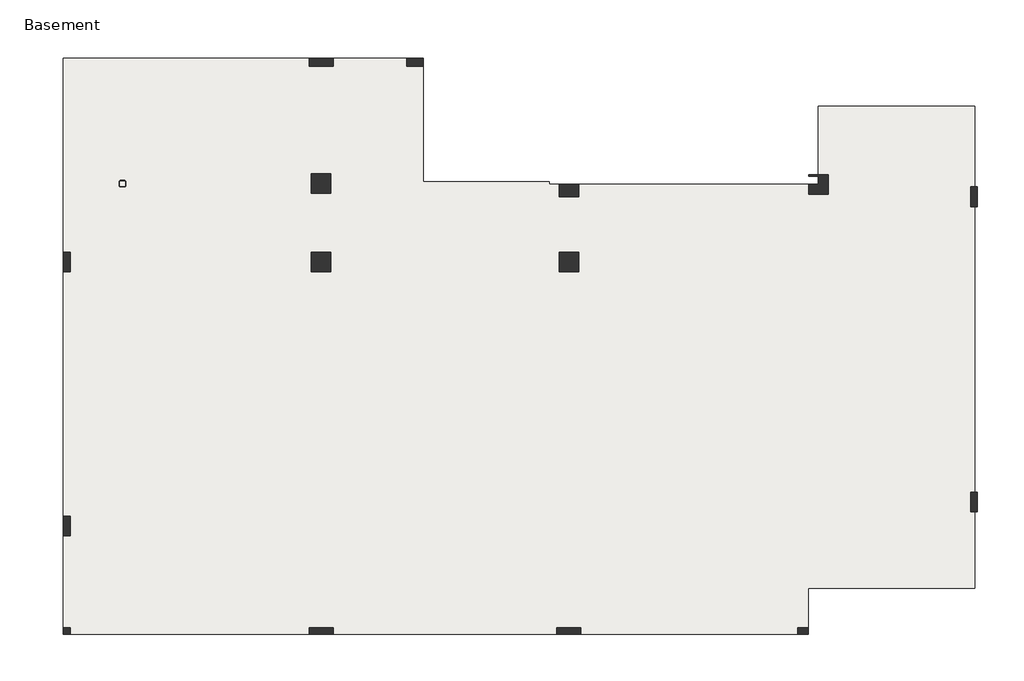
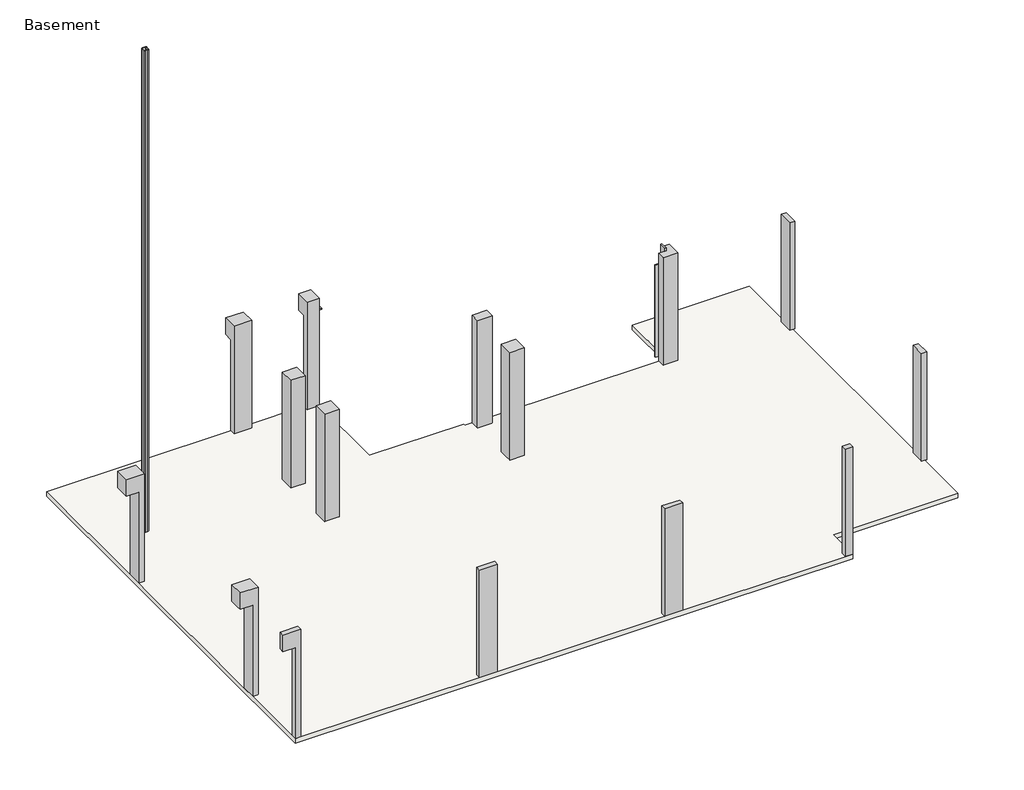
# One storey: 16 columns, 1 slab.
"""IFC4 building model written with IfcOpenShell, lengths in millimetres."""

import ifcopenshell
import ifcopenshell.guid

model = None  # the IFC model being written
_history = None  # IfcOwnerHistory: only IFC2X3 demands one
_inside = {}  # id of a spatial element -> (the spatial element, [elements in it])
_under = {}  # id of a project, library or spatial element -> (it, [spatial elements below it])
_declared = {}  # id of a project -> (the project, [libraries it declares])
_typed = {}  # id of a type object -> (the type object, [elements of that type])
_made_of = {}  # id of a material, layer set ... -> (it, [elements and type objects made of it])


def new_model(schema):
    """Start an empty IFC model of exactly this schema.

    Asked for "IFC4X3", IfcOpenShell would pick the latest addendum, in which some entities
    have other attributes; the version numbers below select the first issue.
    IFC2X3 requires an IfcOwnerHistory on every rooted entity: one is made here for all.
    """
    global model, _history
    if schema == "IFC4X3":
        model = ifcopenshell.file(schema_version=(4, 3, 0, 0))
    else:
        model = ifcopenshell.file(schema=schema)
    _inside.clear()
    _under.clear()
    _declared.clear()
    _typed.clear()
    _made_of.clear()
    _history = None
    if model.schema == "IFC2X3":
        org = make("IfcOrganization", Name="unknown")
        user = make(
            "IfcPersonAndOrganization",
            ThePerson=make("IfcPerson", FamilyName="unknown"),
            TheOrganization=org,
        )
        app = make(
            "IfcApplication",
            ApplicationDeveloper=org,
            Version="unknown",
            ApplicationFullName="unknown",
            ApplicationIdentifier="unknown",
        )
        _history = make(
            "IfcOwnerHistory",
            OwningUser=user,
            OwningApplication=app,
            ChangeAction="ADDED",
            CreationDate=0,
        )
    return model


def make(cls, **values):
    """One entity of the class cls with the attributes given. An attribute that is None is left unset."""
    return model.create_entity(
        cls, **{name: value for name, value in values.items() if value is not None}
    )


def rooted(cls, **values):
    """An entity with a GlobalId (a new one), such as an element, a storey or a relation."""
    return make(cls, GlobalId=ifcopenshell.guid.new(), OwnerHistory=_history, **values)


def si_unit(unit_type, name, prefix=None):
    """IfcSIUnit, for example si_unit("LENGTHUNIT", "METRE", prefix="MILLI")."""
    return make("IfcSIUnit", UnitType=unit_type, Prefix=prefix, Name=name)


def assignment(units):
    """IfcUnitAssignment: the units of a project."""
    return None if units is None else make("IfcUnitAssignment", Units=units)


def point(xyz):
    """IfcCartesianPoint."""
    return None if xyz is None else make("IfcCartesianPoint", Coordinates=xyz)


def direction(xyz):
    """IfcDirection."""
    return None if xyz is None else make("IfcDirection", DirectionRatios=xyz)


def frame(location, z_axis=None, x_axis=None):
    """IfcAxis2Placement3D, a coordinate frame: its origin and axes. An axis left out is left unset."""
    return make(
        "IfcAxis2Placement3D",
        Location=point(location),
        Axis=direction(z_axis),
        RefDirection=direction(x_axis),
    )


def frame_2d(location, x_axis=None):
    """IfcAxis2Placement2D, a coordinate frame in the plane: its origin and x axis."""
    return make(
        "IfcAxis2Placement2D", Location=point(location), RefDirection=direction(x_axis)
    )


def origin():
    """The frame at (0, 0, 0) with its axes left unset."""
    return frame((0.0, 0.0, 0.0))


def place(relative_to, where):
    """IfcLocalPlacement: puts the frame where relative to a parent placement (None: the world)."""
    return make(
        "IfcLocalPlacement", PlacementRelTo=relative_to, RelativePlacement=where
    )


def context(
    kind, dimensions, precision=None, world=None, true_north=None, identifier=None
):
    """IfcGeometricRepresentationContext, for example the 3D "Model" context."""
    return make(
        "IfcGeometricRepresentationContext",
        ContextIdentifier=identifier,
        ContextType=kind,
        CoordinateSpaceDimension=dimensions,
        Precision=precision,
        WorldCoordinateSystem=world,
        TrueNorth=true_north,
    )


def project(units=None, contexts=None):
    """IfcProject with its units and contexts."""
    return rooted(
        "IfcProject",
        Name="project",
        RepresentationContexts=contexts,
        UnitsInContext=assignment(units),
    )


def spatial(cls, under=None, at=None, **own):
    """A site, building, storey or space (cls), placed at a placement, below another one or the project."""
    s = rooted(cls, ObjectPlacement=at, **own)
    if under is not None:
        _under.setdefault(under.id(), (under, []))[1].append(s)
    return s


def polyline(points):
    """IfcPolyline through the points."""
    return make("IfcPolyline", Points=[point(p) for p in points])


def circle_curve(where, radius):
    """IfcCircle in the frame where."""
    return make("IfcCircle", Position=where, Radius=radius)


def trimmed(basis, trim1, trim2, sense, master):
    """IfcTrimmedCurve: the piece of a basis curve between two trims."""
    return make(
        "IfcTrimmedCurve",
        BasisCurve=basis,
        Trim1=trim1,
        Trim2=trim2,
        SenseAgreement=sense,
        MasterRepresentation=master,
    )


def segment(curve, same_sense, transition):
    """IfcCompositeCurveSegment."""
    return make(
        "IfcCompositeCurveSegment",
        Transition=transition,
        SameSense=same_sense,
        ParentCurve=curve,
    )


def composite_curve(segments, self_intersect=None):
    """IfcCompositeCurve: segments joined end to end."""
    return make("IfcCompositeCurve", Segments=segments, SelfIntersect=self_intersect)


def outline(outer, holes=None, kind="AREA"):
    """IfcArbitraryClosedProfileDef: a profile drawn as a closed curve; with holes, ...WithVoids."""
    if holes is None:
        return make("IfcArbitraryClosedProfileDef", ProfileType=kind, OuterCurve=outer)
    return make(
        "IfcArbitraryProfileDefWithVoids",
        ProfileType=kind,
        OuterCurve=outer,
        InnerCurves=holes,
    )


def extrude(swept, where, along, depth):
    """IfcExtrudedAreaSolid: the profile swept, set in the frame where, extruded along a direction by depth."""
    return make(
        "IfcExtrudedAreaSolid",
        SweptArea=swept,
        Position=where,
        ExtrudedDirection=direction(along),
        Depth=depth,
    )


def faces_of(points, faces, orient=None, outer=None):
    """IfcFace entities. A face is a list of loops; a loop is a list of indices into points, from 0.

    orient and outer hold one flag for each loop. By default every Orientation is true, the
    first loop of a face is its IfcFaceOuterBound and the others are IfcFaceBound.
    """
    made = []
    for i, loops in enumerate(faces):
        bounds = []
        for j, loop in enumerate(loops):
            is_outer = j == 0 if outer is None else outer[i][j]
            bounds.append(
                make(
                    "IfcFaceOuterBound" if is_outer else "IfcFaceBound",
                    Bound=make("IfcPolyLoop", Polygon=[points[k] for k in loop]),
                    Orientation=True if orient is None else orient[i][j],
                )
            )
        made.append(make("IfcFace", Bounds=bounds))
    return made


def faceted_brep(points, faces, orient=None, outer=None, voids=None):
    """IfcFacetedBrep: a solid bounded by flat faces; with voids (closed shells), ...WithVoids."""
    shared = [point(p) for p in points]
    hull = make("IfcClosedShell", CfsFaces=faces_of(shared, faces, orient, outer))
    if voids is None:
        return make("IfcFacetedBrep", Outer=hull)
    return make(
        "IfcFacetedBrepWithVoids",
        Outer=hull,
        Voids=[
            make(cls, CfsFaces=faces_of(shared, fs, o, b)) for cls, fs, o, b in voids
        ],
    )


def shape(context_of_items, identifier, shape_type, items):
    """IfcShapeRepresentation: the items that make up one representation, for example the "Body"."""
    return make(
        "IfcShapeRepresentation",
        ContextOfItems=context_of_items,
        RepresentationIdentifier=identifier,
        RepresentationType=shape_type,
        Items=items,
    )


def source(mapping_origin, context_of_items, identifier, shape_type, items):
    """IfcRepresentationMap: a shape defined once, which mapped items show again and again."""
    return make(
        "IfcRepresentationMap",
        MappingOrigin=mapping_origin,
        MappedRepresentation=shape(context_of_items, identifier, shape_type, items),
    )


def transform(
    local_origin,
    x_axis=None,
    y_axis=None,
    z_axis=None,
    scale=None,
    scale2=None,
    scale3=None,
    uniform=True,
):
    """IfcCartesianTransformationOperator3D, or its non-uniform kind. x_axis, y_axis, z_axis: its Axis1, 2, 3."""
    if uniform:
        return make(
            "IfcCartesianTransformationOperator3D",
            Axis1=direction(x_axis),
            Axis2=direction(y_axis),
            LocalOrigin=point(local_origin),
            Scale=scale,
            Axis3=direction(z_axis),
        )
    return make(
        "IfcCartesianTransformationOperator3DnonUniform",
        Axis1=direction(x_axis),
        Axis2=direction(y_axis),
        LocalOrigin=point(local_origin),
        Scale=scale,
        Axis3=direction(z_axis),
        Scale2=scale2,
        Scale3=scale3,
    )


def mapped(mapping_source, mapping_target):
    """IfcMappedItem: shows the shape of a source again, moved by a transform."""
    return make(
        "IfcMappedItem", MappingSource=mapping_source, MappingTarget=mapping_target
    )


def made_of(thing, what):
    """Note that an element or type object is made of a material, layer set ...; save() writes the relation."""
    if what is not None:
        _made_of.setdefault(what.id(), (what, []))[1].append(thing)
    return thing


def element(
    cls,
    number,
    at=None,
    inside=None,
    cuts=None,
    type_object=None,
    material=None,
    context=None,
    identifier="Body",
    shape_type=None,
    held_by="IfcProductDefinitionShape",
    body=None,
    shapes=None,
    **own,
):
    """One element of the class cls, such as IfcWall. Its Tag is "e" and its number.

    at: its placement. inside: the storey or other place that contains it. cuts: it is an
    opening in that element (IfcRelVoidsElement). A single representation is given by context,
    identifier, shape_type and body (its items); several are given by shapes. held_by: the class
    of the entity that holds the representations. save() writes the other relations.
    """
    e = rooted(cls, Tag="e%d" % number, ObjectPlacement=at, **own)
    if body is not None:
        shapes = [shape(context, identifier, shape_type, body)]
    if shapes is not None:
        e.Representation = make(held_by, Representations=shapes)
    if inside is not None:
        _inside.setdefault(inside.id(), (inside, []))[1].append(e)
    if cuts is not None:
        rooted(
            "IfcRelVoidsElement", RelatingBuildingElement=cuts, RelatedOpeningElement=e
        )
    if type_object is not None:
        _typed.setdefault(type_object.id(), (type_object, []))[1].append(e)
    return made_of(e, material)


def aggregate(whole, parts):
    """IfcRelAggregates: a whole, such as a stair, and the parts it consists of."""
    return rooted("IfcRelAggregates", RelatingObject=whole, RelatedObjects=parts)


def save(model, path):
    """Write the relations noted so far, then the file.

    IfcRelAggregates (storeys below a building ...), IfcRelContainedInSpatialStructure (elements
    in a storey), IfcRelDefinesByType, IfcRelAssociatesMaterial and IfcRelDeclares: one each for
    every whole, place, type object, material and project.
    """
    for whole, parts in _under.values():
        aggregate(whole, parts)
    for where, things in _inside.values():
        rooted(
            "IfcRelContainedInSpatialStructure",
            RelatedElements=things,
            RelatingStructure=where,
        )
    for kind, things in _typed.values():
        rooted("IfcRelDefinesByType", RelatedObjects=things, RelatingType=kind)
    for what, things in _made_of.values():
        rooted("IfcRelAssociatesMaterial", RelatedObjects=things, RelatingMaterial=what)
    for by, libraries in _declared.values():
        rooted("IfcRelDeclares", RelatingContext=by, RelatedDefinitions=libraries)
    model.write(path)


def hss_hollow_structural_section_column_hss6x6x5_8_d9445e73(model_context):
    return source(origin(), model_context, "Body", "SweptSolid", [
        extrude(outline(composite_curve([segment(trimmed(circle_curve(frame_2d((46.6852, 46.6852)), 29.5148), [point((46.6852, 76.2))], [point((76.2, 46.6852))], False, "CARTESIAN"), True, "CONTINUOUS"), segment(polyline([(76.2, 46.6852), (76.2, -46.6852)]), True, "CONTINUOUS"), segment(trimmed(circle_curve(frame_2d((46.6852, -46.6852)), 29.5148), [point((76.2, -46.6852))], [point((46.6852, -76.2))], False, "CARTESIAN"), True, "CONTINUOUS"), segment(polyline([(46.6852, -76.2), (-46.6852, -76.2)]), True, "CONTINUOUS"), segment(trimmed(circle_curve(frame_2d((-46.6852, -46.6852)), 29.5148), [point((-46.6852, -76.2))], [point((-76.2, -46.6852))], False, "CARTESIAN"), True, "CONTINUOUS"), segment(polyline([(-76.2, -46.6852), (-76.2, 46.6852)]), True, "CONTINUOUS"), segment(trimmed(circle_curve(frame_2d((-46.6852, 46.6852)), 29.5148), [point((-76.2, 46.6852))], [point((-46.6852, 76.2))], False, "CARTESIAN"), True, "CONTINUOUS"), segment(polyline([(-46.6852, 76.2), (46.6852, 76.2)]), True, "CONTINUOUS")], self_intersect=False), holes=[composite_curve([segment(polyline([(46.6852, 61.4426), (-46.6852, 61.4426)]), True, "CONTINUOUS"), segment(trimmed(circle_curve(frame_2d((-46.6852, 46.6852)), 14.7574), [point((-46.6852, 61.4426))], [point((-61.4426, 46.6852))], True, "CARTESIAN"), True, "CONTINUOUS"), segment(polyline([(-61.4426, 46.6852), (-61.4426, -46.6852)]), True, "CONTINUOUS"), segment(trimmed(circle_curve(frame_2d((-46.6852, -46.6852)), 14.7574), [point((-61.4426, -46.6852))], [point((-46.6852, -61.4426))], True, "CARTESIAN"), True, "CONTINUOUS"), segment(polyline([(-46.6852, -61.4426), (46.6852, -61.4426)]), True, "CONTINUOUS"), segment(trimmed(circle_curve(frame_2d((46.6852, -46.6852)), 14.7574), [point((46.6852, -61.4426))], [point((61.4426, -46.6852))], True, "CARTESIAN"), True, "CONTINUOUS"), segment(polyline([(61.4426, -46.6852), (61.4426, 46.6852)]), True, "CONTINUOUS"), segment(trimmed(circle_curve(frame_2d((46.6852, 46.6852)), 14.7574), [point((61.4426, 46.6852))], [point((46.6852, 61.4426))], True, "CARTESIAN"), True, "CONTINUOUS")], self_intersect=False)]), frame((0.0, 0.0, -3657.6), z_axis=(0.0, 0.0, 1.0), x_axis=(1.0, 0.0, 0.0)), (0.0, 0.0, 1.0), 15925.8),
    ])


model = new_model("IFC4")

# Units and contexts
model_context = context("Model", 3, world=origin())
ifc_project = project(units=[si_unit("LENGTHUNIT", "METRE", prefix="MILLI")], contexts=[model_context])

# Site, building, storey
site = spatial("IfcSite", under=ifc_project)
building = spatial("IfcBuilding", under=site)
storey = spatial("IfcBuildingStorey", under=building, Name="Basement", Elevation=-3657.6)

# Columns
placement = place(None, origin())
element("IfcColumn", 1, ObjectType="Concrete-Rectangular-Column : P1", at=placement, inside=storey, context=model_context, shape_type="SweptSolid", body=[
    extrude(outline(polyline([(718.2325311, -3327.2323339), (718.2325311, -3784.4323339), (261.0325311, -3784.4323339), (261.0325311, -3327.2323339), (718.2325311, -3327.2323339)])), frame((0.0, 0.0, -3657.6), z_axis=(0.0, 0.0, 1.0), x_axis=(1.0, 0.0, 0.0)), (0.0, 0.0, 1.0), 3556.0),
])
element("IfcColumn", 2, ObjectType="Concrete-Rectangular-Column : P1", at=placement, inside=storey, context=model_context, shape_type="SweptSolid", body=[
    extrude(outline(polyline([(718.2325311, -5156.0323339), (718.2325311, -5613.2323339), (261.0325311, -5613.2323339), (261.0325311, -5156.0323339), (718.2325311, -5156.0323339)])), frame((0.0, 0.0, -3657.6), z_axis=(0.0, 0.0, 1.0), x_axis=(1.0, 0.0, 0.0)), (0.0, 0.0, 1.0), 3556.0),
])
element("IfcColumn", 3, ObjectType="Concrete-Rectangular-Column : P1", at=placement, inside=storey, context=model_context, shape_type="SweptSolid", body=[
    extrude(outline(polyline([(6509.4325311, -5156.0323339), (6509.4325311, -5613.2323339), (6052.2325311, -5613.2323339), (6052.2325311, -5156.0323339), (6509.4325311, -5156.0323339)])), frame((0.0, 0.0, -3657.6), z_axis=(0.0, 0.0, 1.0), x_axis=(1.0, 0.0, 0.0)), (0.0, 0.0, 1.0), 3556.0),
])
element("IfcColumn", 4, ObjectType="Concrete-Rectangular-Column : P1", at=placement, inside=storey, context=model_context, shape_type="SweptSolid", body=[
    extrude(outline(polyline([(6509.4325311, -3860.6323339), (6052.2325311, -3860.6323339), (6052.2325311, -3573.4286475), (6509.4325311, -3573.4286475), (6509.4325311, -3860.6323339)])), frame((0.0, 0.0, -3657.6), z_axis=(0.0, 0.0, 1.0), x_axis=(1.0, 0.0, 0.0)), (0.0, 0.0, 1.0), 3556.0),
])
element("IfcColumn", 5, ObjectType="Concrete-Rectangular-Column : P1", at=placement, inside=storey, context=model_context, shape_type="Brep", body=[
    faceted_brep([(12346.6700311, -3344.8286475, -3657.6), (12346.6700311, -3802.0286475, -3657.6), (11889.4700311, -3802.0286475, -3657.6), (11889.4700311, -3573.4286475, -3657.6), (12118.0700311, -3573.4286475, -3657.6), (12118.0700311, -3379.7536475, -3657.6), (11889.4700311, -3379.7536475, -3657.6), (11889.4700311, -3344.8286475, -3657.6), (12346.6700311, -3344.8286475, -101.6), (12346.6700311, -3802.0286475, -101.6), (11889.4700311, -3802.0286475, -101.6), (11889.4700311, -3573.4286475, -101.6), (11889.4700311, -3344.8286475, -609.6), (12079.8362175, -3344.8286475, -609.6), (12079.8362175, -3344.8286475, 0.0), (12118.0700311, -3344.8286475, 0.0), (12118.0700311, -3344.8286475, -101.6), (12118.0700311, -3573.4286475, 0.0), (12079.8362175, -3573.4286475, 0.0), (12118.0700311, -3573.4286475, -101.6), (12079.8362175, -3573.4286475, -101.6), (12079.8362175, -3379.7536475, -609.6), (12079.8362175, -3573.4286475, -609.6), (11889.4700311, -3379.7536475, -609.6), (12118.0700311, -3379.7536475, -609.6), (12118.0700311, -3573.4286475, -609.6)], [[[0, 1, 2, 3, 4, 5, 6, 7]], [[1, 0, 8, 9]], [[2, 1, 9, 10]], [[2, 10, 11, 3]], [[0, 7, 12, 13, 14, 15, 16, 8]], [[17, 15, 14, 18]], [[16, 19, 20, 11, 10, 9, 8]], [[19, 17, 18, 20]], [[17, 19, 16, 15]], [[14, 13, 21, 22, 20, 18]], [[13, 12, 23, 21]], [[24, 21, 23, 6, 5]], [[24, 25, 22, 21]], [[25, 24, 5, 4]], [[12, 7, 6, 23]], [[20, 22, 25, 4, 3, 11]]]),
])
element("IfcColumn", 6, ObjectType="Concrete-Rectangular-Column : P2", at=placement, inside=storey, context=model_context, shape_type="SweptSolid", body=[
    extrude(outline(polyline([(210.2325311, -13936.6286475), (769.0325311, -13936.6286475), (769.0325311, -14089.0286475), (210.2325311, -14089.0286475), (210.2325311, -13936.6286475)])), frame((0.0, 0.0, -3657.6), z_axis=(0.0, 0.0, 1.0), x_axis=(1.0, 0.0, 0.0)), (0.0, 0.0, 1.0), 3556.0),
])
element("IfcColumn", 7, ObjectType="Concrete-Rectangular-Column : P2", at=placement, inside=storey, context=model_context, shape_type="SweptSolid", body=[
    extrude(outline(polyline([(-3657.6, -5375.7354689), (-101.6, -5375.7354689), (-101.6, -5934.5354689), (-647.7, -5934.5354689), (-647.7, -5547.7637825), (-3657.6, -5547.7637825), (-3657.6, -5375.7354689)])), frame((0.0, -14089.0286475, 0.0), z_axis=(0.0, 1.0, 0.0), x_axis=(0.0, 0.0, 1.0)), (0.0, 0.0, 1.0), 152.4),
])
element("IfcColumn", 8, ObjectType="Concrete-Rectangular-Column : P2", at=placement, inside=storey, context=model_context, shape_type="Brep", body=[
    faceted_brep([(-5375.7354689, -11328.2323339, -3657.6), (-5375.7354689, -11785.4323339, -3657.6), (-5547.7637825, -11785.4323339, -3657.6), (-5547.7637825, -11328.2323339, -3657.6), (-5375.7354689, -11328.2323339, -101.6), (-5375.7354689, -11785.4323339, -101.6), (-5934.5354689, -11785.4323339, -101.6), (-5934.5354689, -11785.4323339, -647.7), (-5547.7637825, -11785.4323339, -647.7), (-5934.5354689, -11328.2323339, -101.6), (-5934.5354689, -11328.2323339, -647.7), (-5934.5354689, -11653.6698339, -647.7), (-5547.7637825, -11328.2323339, -647.7), (-5547.7637825, -11653.6698339, -647.7)], [[[0, 1, 2, 3]], [[1, 0, 4, 5]], [[1, 5, 6, 7, 8, 2]], [[6, 9, 10, 11, 7]], [[4, 0, 3, 12, 10, 9]], [[5, 4, 9, 6]], [[8, 13, 12, 3, 2]], [[12, 13, 11, 10]], [[13, 8, 7, 11]]]),
])
element("IfcColumn", 9, ObjectType="Concrete-Rectangular-Column : P2", at=placement, inside=storey, context=model_context, shape_type="Brep", body=[
    faceted_brep([(-5375.7354689, -5156.0323339, -3657.6), (-5375.7354689, -5613.2323339, -3657.6), (-5547.7637825, -5613.2323339, -3657.6), (-5547.7637825, -5156.0323339, -3657.6), (-5375.7354689, -5156.0323339, -101.6), (-5375.7354689, -5613.2323339, -101.6), (-5934.5354689, -5613.2323339, -101.6), (-5934.5354689, -5613.2323339, -647.7), (-5547.7637825, -5613.2323339, -647.7), (-5934.5354689, -5156.0323339, -101.6), (-5934.5354689, -5156.0323339, -647.7), (-5934.5354689, -5414.7948339, -647.7), (-5547.7637825, -5156.0323339, -647.7), (-5547.7637825, -5414.7948339, -647.7)], [[[0, 1, 2, 3]], [[1, 0, 4, 5]], [[1, 5, 6, 7, 8, 2]], [[6, 9, 10, 11, 7]], [[4, 0, 3, 12, 10, 9]], [[5, 4, 9, 6]], [[8, 13, 12, 3, 2]], [[12, 13, 11, 10]], [[13, 8, 7, 11]]]),
])
element("IfcColumn", 10, ObjectType="Concrete-Rectangular-Column : P2", at=placement, inside=storey, context=model_context, shape_type="SweptSolid", body=[
    extrude(outline(polyline([(-804.8286475, -3657.6), (-804.8286475, -101.6), (-347.6286475, -101.6), (-347.6286475, -647.7), (-627.0286475, -647.7), (-627.0286475, -3657.6), (-804.8286475, -3657.6)])), frame((210.2325311, 0.0, 0.0), z_axis=(1.0, 0.0, 0.0), x_axis=(0.0, 1.0, 0.0)), (0.0, 0.0, 1.0), 558.8),
])
element("IfcColumn", 11, ObjectType="Concrete-Rectangular-Column : P2", at=placement, inside=storey, context=model_context, shape_type="Brep", body=[
    faceted_brep([(2496.2325311, -804.8286475, -3657.6), (2496.2325311, -627.0286475, -3657.6), (2877.2325311, -627.0286475, -3657.6), (2877.2325311, -804.8286475, -3657.6), (3055.0325311, -627.0286475, -647.7), (3055.0325311, -347.6286475, -647.7), (3055.0325311, -347.6286475, -609.6), (3055.0325311, -627.0286475, -609.6), (2496.2325311, -804.8286475, -101.6), (2877.2325311, -804.8286475, -101.6), (2496.2325311, -347.6286475, -101.6), (2496.2325311, -347.6286475, -647.7), (2496.2325311, -627.0286475, -647.7), (2877.2325311, -347.6286475, -101.6), (2877.2325311, -347.6286475, -609.6), (2877.2325311, -627.0286475, -647.7), (2877.2325311, -627.0286475, -609.6)], [[[0, 1, 2, 3]], [[4, 5, 6, 7]], [[8, 0, 3, 9]], [[0, 8, 10, 11, 12, 1]], [[10, 13, 14, 6, 5, 11]], [[8, 9, 13, 10]], [[1, 12, 15, 2]], [[5, 4, 15, 12, 11]], [[3, 2, 15, 16, 14, 13, 9]], [[15, 4, 7, 16]], [[14, 16, 7, 6]]]),
])
element("IfcColumn", 12, ObjectType="Concrete-Rectangular-Column : P2", at=placement, inside=storey, context=model_context, shape_type="SweptSolid", body=[
    extrude(outline(polyline([(15678.8325311, -4089.2323339), (15678.8325311, -3632.0323339), (15839.0362175, -3632.0323339), (15839.0362175, -4089.2323339), (15678.8325311, -4089.2323339)])), frame((0.0, 0.0, -3657.6), z_axis=(0.0, 0.0, 1.0), x_axis=(1.0, 0.0, 0.0)), (0.0, 0.0, 1.0), 3556.0),
])
element("IfcColumn", 13, ObjectType="Concrete-Rectangular-Column : P2", at=placement, inside=storey, context=model_context, shape_type="SweptSolid", body=[
    extrude(outline(polyline([(15678.8325311, -11226.6323339), (15678.8325311, -10769.4323339), (15839.0362175, -10769.4323339), (15839.0362175, -11226.6323339), (15678.8325311, -11226.6323339)])), frame((0.0, 0.0, -3657.6), z_axis=(0.0, 0.0, 1.0), x_axis=(1.0, 0.0, 0.0)), (0.0, 0.0, 1.0), 3556.0),
])
element("IfcColumn", 14, ObjectType="Concrete-Rectangular-Column : P2", at=placement, inside=storey, context=model_context, shape_type="SweptSolid", body=[
    extrude(outline(polyline([(6001.4325311, -13936.6286475), (6560.2325311, -13936.6286475), (6560.2325311, -14089.0286475), (6001.4325311, -14089.0286475), (6001.4325311, -13936.6286475)])), frame((0.0, 0.0, -3657.6), z_axis=(0.0, 0.0, 1.0), x_axis=(1.0, 0.0, 0.0)), (0.0, 0.0, 1.0), 3556.0),
])
element("IfcColumn", 15, ObjectType="Concrete-Rectangular-Column : P2", at=placement, inside=storey, context=model_context, shape_type="SweptSolid", body=[
    extrude(outline(polyline([(11640.2325311, -13936.6286475), (11876.6362175, -13936.6286475), (11876.6362175, -14089.0286475), (11640.2325311, -14089.0286475), (11640.2325311, -13936.6286475)])), frame((0.0, 0.0, -3657.6), z_axis=(0.0, 0.0, 1.0), x_axis=(1.0, 0.0, 0.0)), (0.0, 0.0, 1.0), 3556.0),
])
hss_hollow_structural_section_column_hss6x6x5_8_shape = hss_hollow_structural_section_column_hss6x6x5_8_d9445e73(model_context)
element("IfcColumn", 16, ObjectType="HSS-Hollow Structural Section-Column : HSS6X6X5/8", at=placement, inside=storey, context=model_context, shape_type="MappedRepresentation", body=[
    mapped(hss_hollow_structural_section_column_hss6x6x5_8_shape, transform((-4158.5674689, -3555.8323339, 0.0), x_axis=(1.0, 0.0, 0.0), y_axis=(0.0, 1.0, 0.0), z_axis=(0.0, 0.0, 1.0))),
])

# Slab
element("IfcSlab", 17, ObjectType="6\" Concrete", at=placement, inside=storey, context=model_context, shape_type="Brep", body=[
    faceted_brep([(2877.2325311, -627.0286475, -3810.0), (2877.2325311, -3504.2703339, -3810.0), (5823.6325311, -3504.2703339, -3810.0), (5823.6325311, -3573.4286475, -3810.0), (12118.0700311, -3573.4286475, -3810.0), (12118.0700311, -1744.6286475, -3810.0), (15775.6700311, -1744.6286475, -3810.0), (15775.6700311, -13022.2286475, -3810.0), (11876.6362175, -13022.2286475, -3810.0), (11876.6362175, -14089.0286475, -3810.0), (-5547.7637825, -14089.0286475, -3810.0), (-5547.7637825, -627.0286475, -3810.0), (2877.2325311, -627.0286475, -3657.6), (2496.2325311, -627.0286475, -3657.6), (769.0325311, -627.0286475, -3657.6), (210.2325311, -627.0286475, -3657.6), (-5547.7637825, -627.0286475, -3657.6), (-5547.7637825, -5156.0323339, -3657.6), (-5547.7637825, -5613.2323339, -3657.6), (-5547.7637825, -11328.2323339, -3657.6), (-5547.7637825, -11785.4323339, -3657.6), (-5547.7637825, -13936.6286475, -3657.6), (-5547.7637825, -14089.0286475, -3657.6), (-5375.7354689, -14089.0286475, -3657.6), (210.2325311, -14089.0286475, -3657.6), (769.0325311, -14089.0286475, -3657.6), (6001.4325311, -14089.0286475, -3657.6), (6560.2325311, -14089.0286475, -3657.6), (11640.2325311, -14089.0286475, -3657.6), (11876.6362175, -14089.0286475, -3657.6), (11876.6362175, -13936.6286475, -3657.6), (11876.6362175, -13022.2286475, -3657.6), (15775.6700311, -13022.2286475, -3657.6), (15775.6700311, -1744.6286475, -3657.6), (12118.0700311, -1744.6286475, -3657.6), (12118.0700311, -3379.7536475, -3657.6), (12118.0700311, -3573.4286475, -3657.6), (11889.4700311, -3573.4286475, -3657.6), (6509.4325311, -3573.4286475, -3657.6), (6052.2325311, -3573.4286475, -3657.6), (5823.6325311, -3573.4286475, -3657.6), (5823.6325311, -3504.2703339, -3657.6), (2877.2325311, -3504.2703339, -3657.6), (2877.2325311, -804.8286475, -3657.6)], [[[0, 1, 2, 3, 4, 5, 6, 7, 8, 9, 10, 11]], [[12, 13, 14, 15, 16, 17, 18, 19, 20, 21, 22, 23, 24, 25, 26, 27, 28, 29, 30, 31, 32, 33, 34, 35, 36, 37, 38, 39, 40, 41, 42, 43]], [[1, 0, 12, 43, 42]], [[2, 1, 42, 41]], [[3, 2, 41, 40]], [[4, 3, 40, 39, 38, 37, 36]], [[5, 4, 36, 35, 34]], [[6, 5, 34, 33]], [[7, 6, 33, 32]], [[8, 7, 32, 31]], [[9, 8, 31, 30, 29]], [[10, 9, 29, 28, 27, 26, 25, 24, 23, 22]], [[11, 10, 22, 21, 20, 19, 18, 17, 16]], [[0, 11, 16, 15, 14, 13, 12]]]),
])

save(model, "model.ifc")

# Revit data of these elements
# Project information
#   Project Issue Date = "Issue Date"
#   Project Status = "Project Status"
#   Client Name = "Owner"
#   Project Address = "Enter address here"
#   Project Name = "Project Name"
#   Project Number = "Project Number"
# Grids (mm)
#   "1": line (-30549.167, -17339.647) -> (-30549.167, 13720.807)
#   "2": line (-27221.767, -17339.647) -> (-27221.767, 13720.807)
#   "3": line (-21532.167, -17339.647) -> (-21532.167, 13720.807)
#   "4": line (-15842.567, -17339.647) -> (-15842.567, 13720.807)
#   "5": line (-9848.167, -17339.647) -> (-9848.167, 13720.807)
#   "7": line (-4158.567, -17339.647) -> (-4158.567, 13720.807)
#   "8": line (489.633, -17339.647) -> (489.633, 13720.807)
#   "10": line (12072.033, -17339.647) -> (12072.033, 1480.434)
#   "11": line (16034.433, -17339.647) -> (16034.433, 1480.434)
#   "A": line (23085.988, -14300.032) -> (-7127.732, -14300.032)
#   "D": line (23085.988, -5384.632) -> (-7127.732, -5384.632)
#   "E": line (23085.988, -3555.832) -> (-30549.167, -3555.832)
#   "F": line (23085.988, -431.632) -> (-7127.732, -431.632)
#   "B": line (23085.988, -11556.832) -> (-30549.167, -11556.832)
#   "G": line (1892.436, 4775.368) -> (-30549.167, 4775.368)
#   "H": line (1892.436, 9118.768) -> (-30549.167, 9118.768)
#   "C": line (23085.988, -9169.232) -> (-7127.732, -9169.232)
#   "6": line (-5758.767, -17339.647) -> (-5758.767, -2380.252)
#   "9": line (6280.833, -17339.647) -> (6280.833, 1480.434)
# Type "Concrete-Rectangular-Column : P1"
#   Assembly Code = "B10"
#   b = 1' - 6"
#   h = 1' - 6"
#   Structural Material [instance default] = Concrete, Cast-in-Place gray
# Type "Concrete-Rectangular-Column : P2"
#   Assembly Code = "B10"
#   b = 1' - 10"
#   h = 1' - 6"
#   Structural Material [instance default] = Concrete, Cast-in-Place gray
# Type "HSS-Hollow Structural Section-Column : HSS6X6X5/8"
#   Assembly Code = "B10"
#   Shape = "Square"
#   W = 42.1
#   Ht = 0' - 6"
#   b = 0' - 6"
#   kr = 0' - 1.162"
#   t = 0' - 0.581"
#   A = 0.08125 SF
#   Structural Material [instance default] = Steel ASTM A500, Grade B, Rectangular and Square
# Type "6\" Concrete"
#   Assembly Code = "B1010"
#   Function = 0
#   Layers, outside or top first: 0' - 6" "Concrete, Cast-in-Place gray" (function 1)
# Elements 1, 2, 3, 4, 5 (IfcColumn, "Concrete-Rectangular-Column : P1")
#   Comments = ""
#   Structural Material = Concrete, Cast-in-Place gray
#   Phase Created = New Construction
#   Materials on its faces: "Concrete, Cast-in-Place gray"
# Elements 6, 7, 8, 9, 10, 11, 12, 13, 14, 15 (IfcColumn, "Concrete-Rectangular-Column : P2")
#   Comments = ""
#   Structural Material = Concrete, Cast-in-Place gray
#   Phase Created = New Construction
#   Materials on its faces: "Concrete, Cast-in-Place gray"
# Element 16 (IfcColumn, "HSS-Hollow Structural Section-Column : HSS6X6X5/8")
#   Comments = ""
#   Structural Material = Steel ASTM A500, Grade B, Rectangular and Square
#   Phase Created = New Construction
#   Materials on its faces: "Steel ASTM A500, Grade B, Rectangular and Square"
# Element 17 (IfcSlab, "6\" Concrete")
#   Height Offset From Level = 0' - 0"
#   built-in parameter 1001954 = 1
#   Phase Created = New Construction
#   Materials on its faces: "Concrete, Cast-in-Place gray"
# Materials
#   "Concrete, Cast-in-Place gray": class "Concrete", colour RGB 192 192 192, transparency 0, Description = "Cast-in-place concrete", Cost = 0
#   "Steel ASTM A500, Grade B, Rectangular and Square": class "Metal", colour RGB 199 199 199, transparency 0, Description = "Carbon steel", Cost = 0
